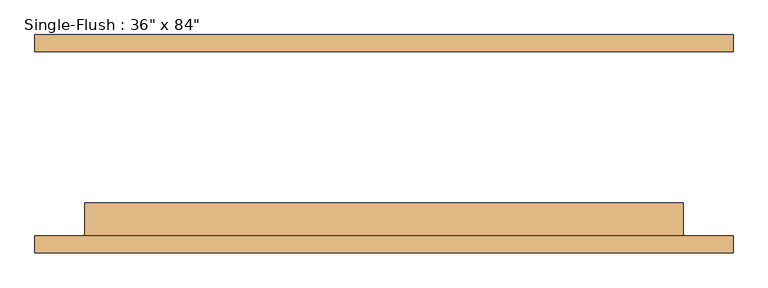
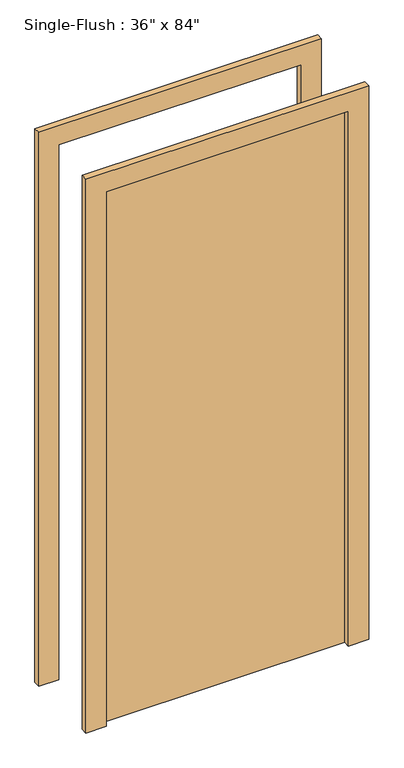
"""IFC4 building model written with IfcOpenShell, lengths in millimetres: door geometry."""

from ifc_helpers import new_model, si_unit, frame, origin, origin_with_axes, place, context, project, spatial, polyline, outline, extrude, source, transform, mapped, element, save


def door_bcc5cfd6(model_context):
    return source(origin(), model_context, "Body", "SweptSolid", [
        extrude(outline(polyline([(2209.8, -533.4), (0.0, -533.4), (0.0, -457.2), (2133.6, -457.2), (2133.6, 457.2), (0.0, 457.2), (0.0, 533.4), (2209.8, 533.4), (2209.8, -533.4)])), frame((0.0, -166.6875, 0.0), z_axis=(0.0, 1.0, 0.0), x_axis=(0.0, 0.0, 1.0)), (0.0, 0.0, 1.0), 25.4),
        extrude(outline(polyline([(2209.8, 533.4), (2209.8, -533.4), (0.0, -533.4), (0.0, -457.2), (2133.6, -457.2), (2133.6, 457.2), (0.0, 457.2), (0.0, 533.4), (2209.8, 533.4)])), frame((0.0, 141.2875, 0.0), z_axis=(0.0, 1.0, 0.0), x_axis=(0.0, 0.0, 1.0)), (0.0, 0.0, 1.0), 25.4),
        extrude(outline(polyline([(457.2, -90.4875), (457.2, -141.2875), (-457.2, -141.2875), (-457.2, -90.4875), (457.2, -90.4875)])), origin_with_axes(), (0.0, 0.0, 1.0), 2133.6),
    ])


if __name__ == "__main__":
    model = new_model("IFC4")
    model_context = context("Model", 3, world=origin())
    ifc_project = project(units=[si_unit("LENGTHUNIT", "METRE", prefix="MILLI")], contexts=[model_context])
    site = spatial("IfcSite", under=ifc_project)
    building = spatial("IfcBuilding", under=site)
    placement = place(None, origin())
    door_shape = door_bcc5cfd6(model_context)
    element("IfcDoor", 1, ObjectType="Single-Flush : 36\" x 84\"", at=placement, inside=building, context=model_context, shape_type="MappedRepresentation", body=[
        mapped(door_shape, transform((0.0, 0.0, 0.0), x_axis=(1.0, 0.0, 0.0), y_axis=(0.0, 1.0, 0.0), z_axis=(0.0, 0.0, 1.0))),
    ])
    save(model, "model.ifc")

# Revit data of these elements
# Type "Single-Flush : 36\" x 84\""
#   Type Mark = "1"
#   Assembly Code = "C1020"
#   Thickness = 0' - 2"
#   Height = 7' - 0"
#   Trim Projection Ext = 0' - 1"
#   Trim Projection Int = 0' - 1"
#   Trim Width = 0' - 3"
#   Width = 3' - 0"
#   Door Material = PAINTED STEEL C CHANNEL
#   Frame Material = PAINTED STEEL C CHANNEL
#   Function = (empty or 0)
#   Wall Closure = (empty or 0)
# Element 1 (IfcDoor, "Single-Flush : 36\" x 84\"")
#   Materials on its faces: "PAINTED STEEL C CHANNEL"
# Materials
#   "PAINTED STEEL C CHANNEL": class "Generic", colour RGB 88 62 61, transparency 0, Cost = 0
